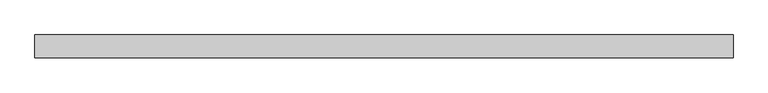
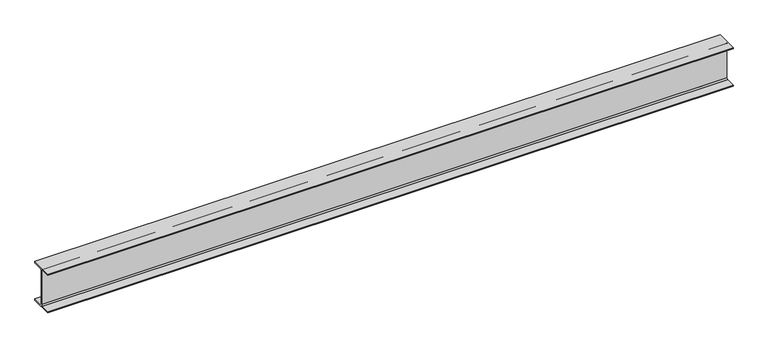
"""IFC4 building model written with IfcOpenShell, lengths in millimetres: beam geometry, Old_Steel Beam_H-KSD3502 : H_SB_ASB_H-300×300x10x15."""

import ifcopenshell
import ifcopenshell.guid

model = None  # the IFC model being written
_history = None  # IfcOwnerHistory: only IFC2X3 demands one
_inside = {}  # id of a spatial element -> (the spatial element, [elements in it])
_under = {}  # id of a project, library or spatial element -> (it, [spatial elements below it])
_declared = {}  # id of a project -> (the project, [libraries it declares])
_typed = {}  # id of a type object -> (the type object, [elements of that type])
_made_of = {}  # id of a material, layer set ... -> (it, [elements and type objects made of it])


def new_model(schema):
    """Start an empty IFC model of exactly this schema.

    Asked for "IFC4X3", IfcOpenShell would pick the latest addendum, in which some entities
    have other attributes; the version numbers below select the first issue.
    IFC2X3 requires an IfcOwnerHistory on every rooted entity: one is made here for all.
    """
    global model, _history
    if schema == "IFC4X3":
        model = ifcopenshell.file(schema_version=(4, 3, 0, 0))
    else:
        model = ifcopenshell.file(schema=schema)
    _inside.clear()
    _under.clear()
    _declared.clear()
    _typed.clear()
    _made_of.clear()
    _history = None
    if model.schema == "IFC2X3":
        org = make("IfcOrganization", Name="unknown")
        user = make(
            "IfcPersonAndOrganization",
            ThePerson=make("IfcPerson", FamilyName="unknown"),
            TheOrganization=org,
        )
        app = make(
            "IfcApplication",
            ApplicationDeveloper=org,
            Version="unknown",
            ApplicationFullName="unknown",
            ApplicationIdentifier="unknown",
        )
        _history = make(
            "IfcOwnerHistory",
            OwningUser=user,
            OwningApplication=app,
            ChangeAction="ADDED",
            CreationDate=0,
        )
    return model


def make(cls, **values):
    """One entity of the class cls with the attributes given. An attribute that is None is left unset."""
    return model.create_entity(
        cls, **{name: value for name, value in values.items() if value is not None}
    )


def rooted(cls, **values):
    """An entity with a GlobalId (a new one), such as an element, a storey or a relation."""
    return make(cls, GlobalId=ifcopenshell.guid.new(), OwnerHistory=_history, **values)


def si_unit(unit_type, name, prefix=None):
    """IfcSIUnit, for example si_unit("LENGTHUNIT", "METRE", prefix="MILLI")."""
    return make("IfcSIUnit", UnitType=unit_type, Prefix=prefix, Name=name)


def assignment(units):
    """IfcUnitAssignment: the units of a project."""
    return None if units is None else make("IfcUnitAssignment", Units=units)


def point(xyz):
    """IfcCartesianPoint."""
    return None if xyz is None else make("IfcCartesianPoint", Coordinates=xyz)


def direction(xyz):
    """IfcDirection."""
    return None if xyz is None else make("IfcDirection", DirectionRatios=xyz)


def frame(location, z_axis=None, x_axis=None):
    """IfcAxis2Placement3D, a coordinate frame: its origin and axes. An axis left out is left unset."""
    return make(
        "IfcAxis2Placement3D",
        Location=point(location),
        Axis=direction(z_axis),
        RefDirection=direction(x_axis),
    )


def frame_2d(location, x_axis=None):
    """IfcAxis2Placement2D, a coordinate frame in the plane: its origin and x axis."""
    return make(
        "IfcAxis2Placement2D", Location=point(location), RefDirection=direction(x_axis)
    )


def origin():
    """The frame at (0, 0, 0) with its axes left unset."""
    return frame((0.0, 0.0, 0.0))


def place(relative_to, where):
    """IfcLocalPlacement: puts the frame where relative to a parent placement (None: the world)."""
    return make(
        "IfcLocalPlacement", PlacementRelTo=relative_to, RelativePlacement=where
    )


def context(
    kind, dimensions, precision=None, world=None, true_north=None, identifier=None
):
    """IfcGeometricRepresentationContext, for example the 3D "Model" context."""
    return make(
        "IfcGeometricRepresentationContext",
        ContextIdentifier=identifier,
        ContextType=kind,
        CoordinateSpaceDimension=dimensions,
        Precision=precision,
        WorldCoordinateSystem=world,
        TrueNorth=true_north,
    )


def project(units=None, contexts=None):
    """IfcProject with its units and contexts."""
    return rooted(
        "IfcProject",
        Name="project",
        RepresentationContexts=contexts,
        UnitsInContext=assignment(units),
    )


def spatial(cls, under=None, at=None, **own):
    """A site, building, storey or space (cls), placed at a placement, below another one or the project."""
    s = rooted(cls, ObjectPlacement=at, **own)
    if under is not None:
        _under.setdefault(under.id(), (under, []))[1].append(s)
    return s


def polyline(points):
    """IfcPolyline through the points."""
    return make("IfcPolyline", Points=[point(p) for p in points])


def circle_curve(where, radius):
    """IfcCircle in the frame where."""
    return make("IfcCircle", Position=where, Radius=radius)


def trimmed(basis, trim1, trim2, sense, master):
    """IfcTrimmedCurve: the piece of a basis curve between two trims."""
    return make(
        "IfcTrimmedCurve",
        BasisCurve=basis,
        Trim1=trim1,
        Trim2=trim2,
        SenseAgreement=sense,
        MasterRepresentation=master,
    )


def segment(curve, same_sense, transition):
    """IfcCompositeCurveSegment."""
    return make(
        "IfcCompositeCurveSegment",
        Transition=transition,
        SameSense=same_sense,
        ParentCurve=curve,
    )


def composite_curve(segments, self_intersect=None):
    """IfcCompositeCurve: segments joined end to end."""
    return make("IfcCompositeCurve", Segments=segments, SelfIntersect=self_intersect)


def outline(outer, holes=None, kind="AREA"):
    """IfcArbitraryClosedProfileDef: a profile drawn as a closed curve; with holes, ...WithVoids."""
    if holes is None:
        return make("IfcArbitraryClosedProfileDef", ProfileType=kind, OuterCurve=outer)
    return make(
        "IfcArbitraryProfileDefWithVoids",
        ProfileType=kind,
        OuterCurve=outer,
        InnerCurves=holes,
    )


def extrude(swept, where, along, depth):
    """IfcExtrudedAreaSolid: the profile swept, set in the frame where, extruded along a direction by depth."""
    return make(
        "IfcExtrudedAreaSolid",
        SweptArea=swept,
        Position=where,
        ExtrudedDirection=direction(along),
        Depth=depth,
    )


def shape(context_of_items, identifier, shape_type, items):
    """IfcShapeRepresentation: the items that make up one representation, for example the "Body"."""
    return make(
        "IfcShapeRepresentation",
        ContextOfItems=context_of_items,
        RepresentationIdentifier=identifier,
        RepresentationType=shape_type,
        Items=items,
    )


def source(mapping_origin, context_of_items, identifier, shape_type, items):
    """IfcRepresentationMap: a shape defined once, which mapped items show again and again."""
    return make(
        "IfcRepresentationMap",
        MappingOrigin=mapping_origin,
        MappedRepresentation=shape(context_of_items, identifier, shape_type, items),
    )


def transform(
    local_origin,
    x_axis=None,
    y_axis=None,
    z_axis=None,
    scale=None,
    scale2=None,
    scale3=None,
    uniform=True,
):
    """IfcCartesianTransformationOperator3D, or its non-uniform kind. x_axis, y_axis, z_axis: its Axis1, 2, 3."""
    if uniform:
        return make(
            "IfcCartesianTransformationOperator3D",
            Axis1=direction(x_axis),
            Axis2=direction(y_axis),
            LocalOrigin=point(local_origin),
            Scale=scale,
            Axis3=direction(z_axis),
        )
    return make(
        "IfcCartesianTransformationOperator3DnonUniform",
        Axis1=direction(x_axis),
        Axis2=direction(y_axis),
        LocalOrigin=point(local_origin),
        Scale=scale,
        Axis3=direction(z_axis),
        Scale2=scale2,
        Scale3=scale3,
    )


def mapped(mapping_source, mapping_target):
    """IfcMappedItem: shows the shape of a source again, moved by a transform."""
    return make(
        "IfcMappedItem", MappingSource=mapping_source, MappingTarget=mapping_target
    )


def made_of(thing, what):
    """Note that an element or type object is made of a material, layer set ...; save() writes the relation."""
    if what is not None:
        _made_of.setdefault(what.id(), (what, []))[1].append(thing)
    return thing


def element(
    cls,
    number,
    at=None,
    inside=None,
    cuts=None,
    type_object=None,
    material=None,
    context=None,
    identifier="Body",
    shape_type=None,
    held_by="IfcProductDefinitionShape",
    body=None,
    shapes=None,
    **own,
):
    """One element of the class cls, such as IfcWall. Its Tag is "e" and its number.

    at: its placement. inside: the storey or other place that contains it. cuts: it is an
    opening in that element (IfcRelVoidsElement). A single representation is given by context,
    identifier, shape_type and body (its items); several are given by shapes. held_by: the class
    of the entity that holds the representations. save() writes the other relations.
    """
    e = rooted(cls, Tag="e%d" % number, ObjectPlacement=at, **own)
    if body is not None:
        shapes = [shape(context, identifier, shape_type, body)]
    if shapes is not None:
        e.Representation = make(held_by, Representations=shapes)
    if inside is not None:
        _inside.setdefault(inside.id(), (inside, []))[1].append(e)
    if cuts is not None:
        rooted(
            "IfcRelVoidsElement", RelatingBuildingElement=cuts, RelatedOpeningElement=e
        )
    if type_object is not None:
        _typed.setdefault(type_object.id(), (type_object, []))[1].append(e)
    return made_of(e, material)


def aggregate(whole, parts):
    """IfcRelAggregates: a whole, such as a stair, and the parts it consists of."""
    return rooted("IfcRelAggregates", RelatingObject=whole, RelatedObjects=parts)


def save(model, path):
    """Write the relations noted so far, then the file.

    IfcRelAggregates (storeys below a building ...), IfcRelContainedInSpatialStructure (elements
    in a storey), IfcRelDefinesByType, IfcRelAssociatesMaterial and IfcRelDeclares: one each for
    every whole, place, type object, material and project.
    """
    for whole, parts in _under.values():
        aggregate(whole, parts)
    for where, things in _inside.values():
        rooted(
            "IfcRelContainedInSpatialStructure",
            RelatedElements=things,
            RelatingStructure=where,
        )
    for kind, things in _typed.values():
        rooted("IfcRelDefinesByType", RelatedObjects=things, RelatingType=kind)
    for what, things in _made_of.values():
        rooted("IfcRelAssociatesMaterial", RelatedObjects=things, RelatingMaterial=what)
    for by, libraries in _declared.values():
        rooted("IfcRelDeclares", RelatingContext=by, RelatedDefinitions=libraries)
    model.write(path)


def beam_536b1723(model_context):
    return source(origin(), model_context, "Body", "SweptSolid", [
        extrude(outline(composite_curve([segment(polyline([(82.5, -141.5), (82.5, -151.7), (-82.5, -151.7), (-82.5, -141.5), (-11.9, -141.5)]), True, "CONTINUOUS"), segment(trimmed(circle_curve(frame_2d((-11.9, -132.6)), 8.9), [point((-11.9, -141.5))], [point((-3.0, -132.6))], True, "CARTESIAN"), True, "CONTINUOUS"), segment(polyline([(-3.0, -132.6), (-3.0, 132.6)]), True, "CONTINUOUS"), segment(trimmed(circle_curve(frame_2d((-11.9, 132.6)), 8.9), [point((-3.0, 132.6))], [point((-11.9, 141.5))], True, "CARTESIAN"), True, "CONTINUOUS"), segment(polyline([(-11.9, 141.5), (-82.5, 141.5), (-82.5, 151.7), (82.5, 151.7), (82.5, 141.5), (11.9, 141.5)]), True, "CONTINUOUS"), segment(trimmed(circle_curve(frame_2d((11.9, 132.6)), 8.9), [point((11.9, 141.5))], [point((3.0, 132.6))], True, "CARTESIAN"), True, "CONTINUOUS"), segment(polyline([(3.0, 132.6), (3.0, -132.6)]), True, "CONTINUOUS"), segment(trimmed(circle_curve(frame_2d((11.9, -132.6)), 8.9), [point((3.0, -132.6))], [point((11.9, -141.5))], True, "CARTESIAN"), True, "CONTINUOUS"), segment(polyline([(11.9, -141.5), (82.5, -141.5)]), True, "CONTINUOUS")], self_intersect=False)), frame((-2413.6981883, 0.0, 0.0), z_axis=(1.0, 0.0, 0.0), x_axis=(0.0, 1.0, 0.0)), (0.0, 0.0, 1.0), 5076.9152279),
    ])


if __name__ == "__main__":
    model = new_model("IFC4")
    model_context = context("Model", 3, world=origin())
    ifc_project = project(units=[si_unit("LENGTHUNIT", "METRE", prefix="MILLI")], contexts=[model_context])
    site = spatial("IfcSite", under=ifc_project)
    building = spatial("IfcBuilding", under=site)
    placement = place(None, origin())
    beam_shape = beam_536b1723(model_context)
    element("IfcBeam", 1, ObjectType="Old_Steel Beam_H-KSD3502 : H_SB_ASB_H-300×300x10x15", at=placement, inside=building, context=model_context, shape_type="MappedRepresentation", body=[
        mapped(beam_shape, transform((0.0, 0.0, 0.0), x_axis=(1.0, 0.0, 0.0), y_axis=(0.0, 1.0, 0.0), z_axis=(0.0, 0.0, 1.0))),
    ])
    save(model, "model.ifc")

# Revit data of these elements
# Type "Old_Steel Beam_H-KSD3502 : H_SB_ASB_H-300×300x10x15"
#   Width = 30.0 cm
#   Web Thickness = 1.0 cm
#   Web Fillet = 1.8 cm
#   Warping Constant = 1370670.0 cm⁶
#   Torsional Moment of Inertia = 77.00 cm⁴
#   Torsional Modulus = 1.0 cm³
#   Section Area = 119.8 cm²
#   Plastic Modulus weak axis = 684.0 cm³
#   Plastic Modulus strong axis = 1500.0 cm³
#   Perimeter = 1.75 m²/m
#   Nominal Weight = 94.00 kgf/m
#   Moment of Inertia weak axis = 6750.00 cm⁴
#   Moment of Inertia strong axis = 20400.00 cm⁴
#   Height = 30.0 cm
#   Flange Thickness = 1.5 cm
#   Elastic Modulus weak axis = 450.0 cm³
#   Elastic Modulus strong axis = 1360.0 cm³
#   Centroid Vertical = 15.0 cm
#   Centroid Horizontal = 15.0 cm
#   Length [instance default] = 1.5240 m
#   Structural Material [instance default] = Steel, 45-345
#   Assembly Code = ""
# Element 1 (IfcBeam, "Old_Steel Beam_H-KSD3502 : H_SB_ASB_H-300×300x10x15")
#   Structural Material = none
# Materials
#   "Steel, 45-345": class "Metal", colour RGB 189 187 185, transparency 0, Description = "Steel 345 MPa", Cost = 0
